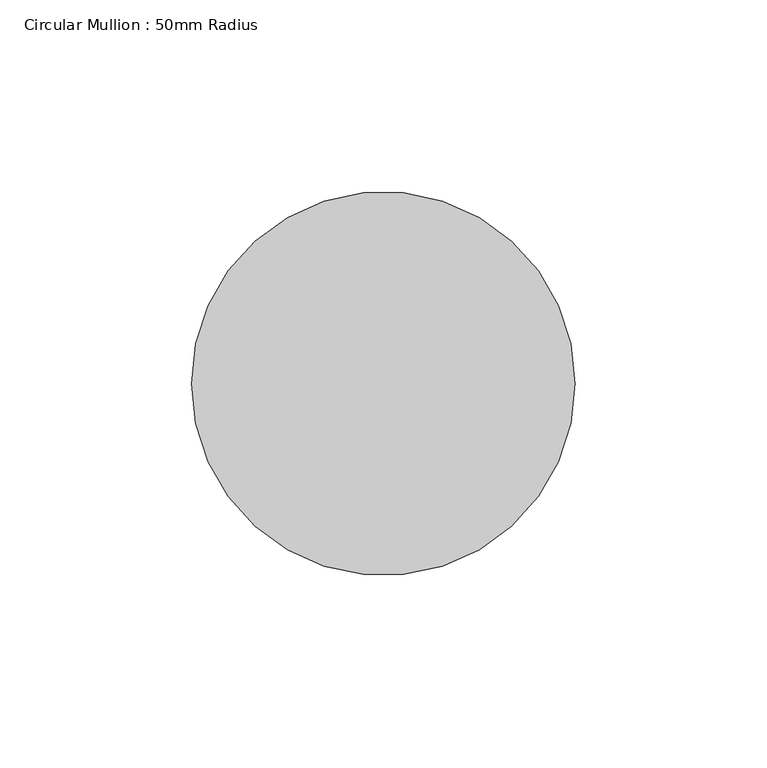
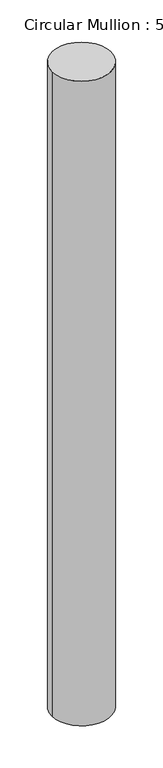
"""IFC4 building model written with IfcOpenShell, lengths in millimetres: member geometry, Circular Mullion : 50mm Radius."""

from ifc_helpers import new_model, si_unit, point, frame, origin, origin_2d, place, context, project, spatial, circle_curve, trimmed, segment, composite_curve, outline, extrude, source, transform, mapped, element, save


def circular_mullion_50mm_radius_b667a65b(model_context):
    return source(origin(), model_context, "Body", "SweptSolid", [
        extrude(outline(composite_curve([segment(trimmed(circle_curve(origin_2d(), 50.0), [point((50.0, 0.0))], [point((-50.0, 0.0))], False, "CARTESIAN"), True, "CONTINUOUS"), segment(trimmed(circle_curve(origin_2d(), 50.0), [point((-50.0, 0.0))], [point((50.0, 0.0))], False, "CARTESIAN"), True, "CONTINUOUS")], self_intersect=False)), frame((0.0, 0.0, -1149.21591), z_axis=(0.0, 0.0, 1.0), x_axis=(1.0, 0.0, 0.0)), (0.0, 0.0, 1.0), 1149.21591),
    ])


if __name__ == "__main__":
    model = new_model("IFC4")
    model_context = context("Model", 3, world=origin())
    ifc_project = project(units=[si_unit("LENGTHUNIT", "METRE", prefix="MILLI")], contexts=[model_context])
    site = spatial("IfcSite", under=ifc_project)
    building = spatial("IfcBuilding", under=site)
    placement = place(None, origin())
    circular_mullion_50mm_radius_shape = circular_mullion_50mm_radius_b667a65b(model_context)
    element("IfcMember", 1, ObjectType="Circular Mullion : 50mm Radius", at=placement, inside=building, context=model_context, shape_type="MappedRepresentation", body=[
        mapped(circular_mullion_50mm_radius_shape, transform((0.0, 0.0, 0.0), x_axis=(1.0, 0.0, 0.0), y_axis=(0.0, 1.0, 0.0), z_axis=(0.0, 0.0, 1.0))),
    ])
    save(model, "model.ifc")

# Revit data of these elements
# Type "Circular Mullion : 50mm Radius"
#   built-in parameter 1007350 = 0.164042 (stored number, unit not read)
# Element 1 (IfcMember, "Circular Mullion : 50mm Radius")
#   Materials on its faces: "Aluminium"
# Materials
#   "Aluminium": class "Metal", colour RGB 247 247 247, transparency 0, Description = "Aluminium 6061", Cost = 0
